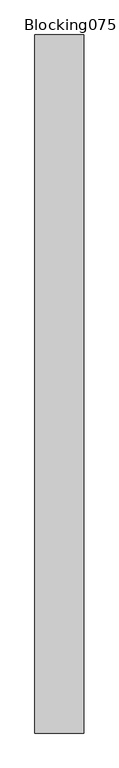
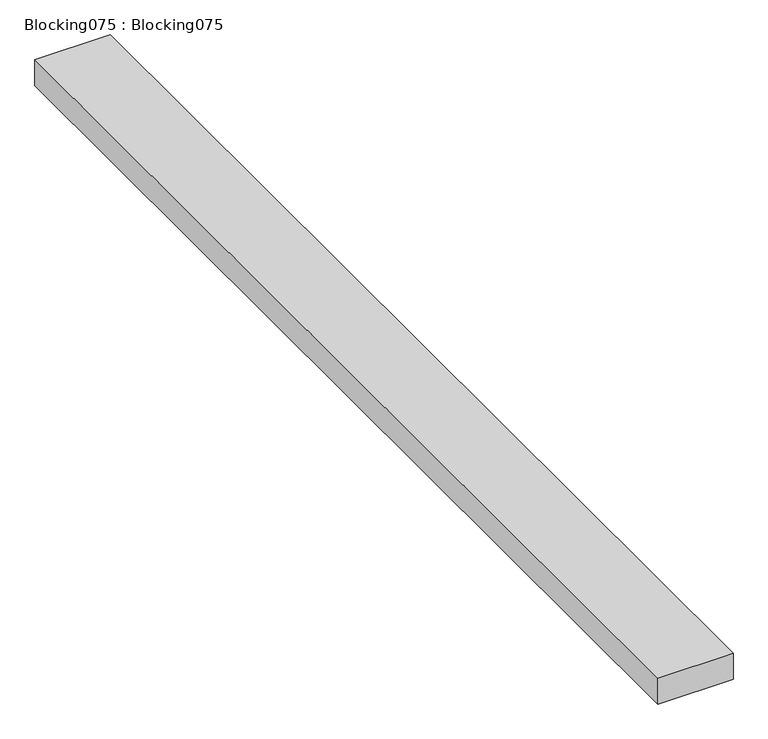
"""IFC4 building model written with IfcOpenShell, lengths in millimetres: proxy geometry, Blocking075 : Blocking075."""

from ifc_helpers import new_model, si_unit, frame, origin, place, context, project, spatial, polyline, outline, extrude, source, transform, mapped, element, save


def blocking075_blocking075_b43752c3(model_context):
    return source(origin(), model_context, "Body", "SweptSolid", [
        extrude(outline(polyline([(-950.3815411, -1052.8908936), (-1090.0815411, -1052.8908936), (-1090.0815411, 947.1091064), (-950.3815411, 947.1091064), (-950.3815411, -1052.8908936)])), frame((0.0, 0.0, 42032.2036692), z_axis=(0.0, 0.0, 1.0), x_axis=(1.0, 0.0, 0.0)), (0.0, 0.0, 1.0), 50.8),
    ])


if __name__ == "__main__":
    model = new_model("IFC4")
    model_context = context("Model", 3, world=origin())
    ifc_project = project(units=[si_unit("LENGTHUNIT", "METRE", prefix="MILLI")], contexts=[model_context])
    site = spatial("IfcSite", under=ifc_project)
    building = spatial("IfcBuilding", under=site)
    placement = place(None, origin())
    blocking075_blocking075_shape = blocking075_blocking075_b43752c3(model_context)
    element("IfcBuildingElementProxy", 1, Name="Blocking075 : Blocking075", ObjectType="Blocking075 : Blocking075", at=placement, inside=building, context=model_context, shape_type="MappedRepresentation", body=[
        mapped(blocking075_blocking075_shape, transform((0.0, 0.0, 0.0), x_axis=(1.0, 0.0, 0.0), y_axis=(0.0, 1.0, 0.0), z_axis=(0.0, 0.0, 1.0))),
    ])
    save(model, "model.ifc")

# Revit data of these elements
# Type "Blocking075 : Blocking075"
#   NameOverride = "Blocking075"
# Element 1 (IfcBuildingElementProxy, "Blocking075 : Blocking075")
#   Materials on its faces: "WOOD BLOCKING AS REQUIRED"
# Materials
#   "WOOD BLOCKING AS REQUIRED": class "Unassigned", colour RGB 166 124 85, transparency 0, Cost = 0
